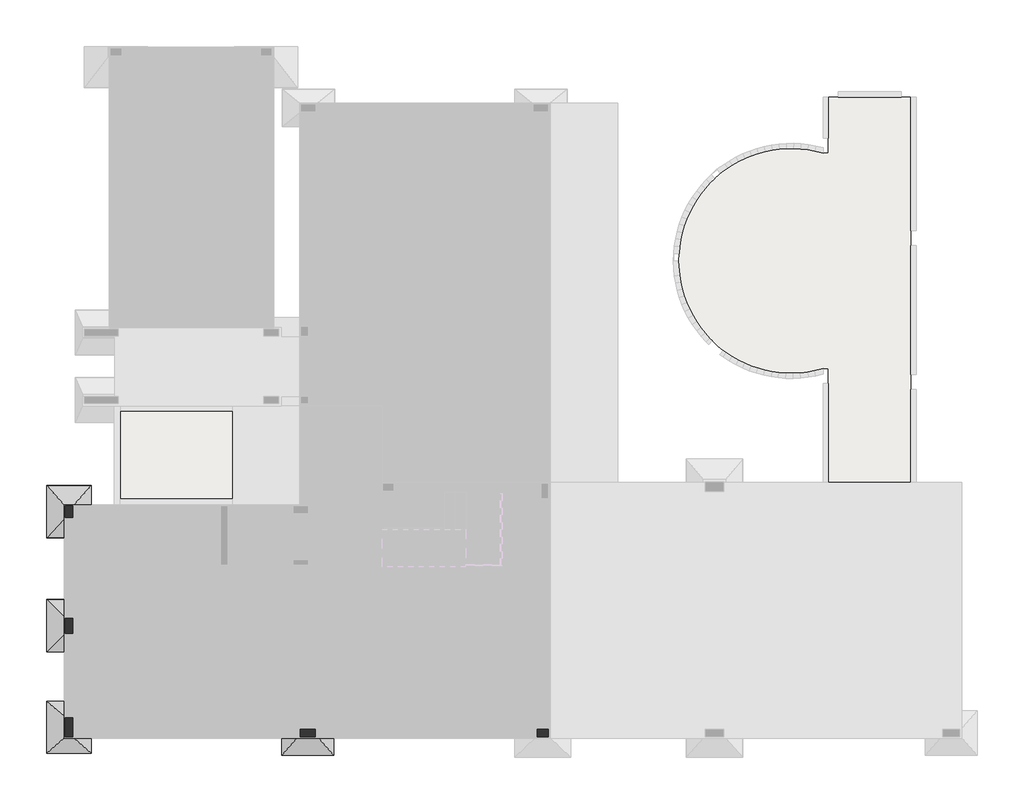
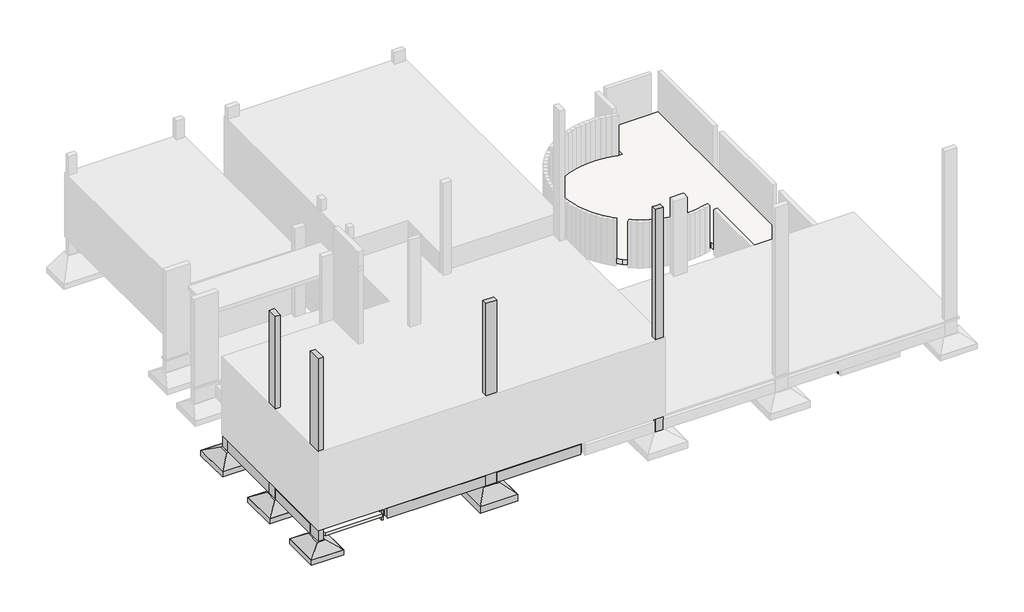
# One storey, part 1 of 4: 11 beams, 5 columns, 4 fasteners, 3 slabs.
# Revit data of these elements (continued)
# Project information
#   Design Option = "Main Model"
#   Project Status = "Status do projeto"
#   Project Address = "RUA SÉRGIO DIAS, LOTE 30, QUADRA G, MONTE MINEIRO/MG"
#   Project Name = "RESIDÊNCIA - ROBERTA VENDRAMINI"
#   Project Number = "034/2017"
#   Zona = "ZER - 01"
#   CA Mín = "0.2"
#   CA Básico = "1"
#   CA Máx = "2"
#   TO Máx = "50"
#   Gabarito Máx = "10"
#   TP Mín = "15"
#   Área Total do Terreno = "620.00 m²"
#   Multifamiliar - Vagas Veículos/Pavto = "0"
#   Multifamiliar - Vagas Bicicletas/Pavto = "0"
#   Multifamiliar - % Vagas PNMR = "0"
#   Multifamiliar - % Vagas Motos = "0"
#   Outros - Área p/ 1 Veículo = "0.00 m²"
#   Outros - Área p/ 1 Bicicleta = "0.00 m²"
#   Outros - Área p/ 1 Utilitário = "0.00 m²"
#   Outros - % Vagas PNMR = "0"
#   Outros - % Vagas Motos = "0"
# Type "TQS - Viga retangular : 14.0 x 40.0"
#   Length [instance default] = 1.524 m
#   b = 0.14 m
#   h = 0.40 m
#   Structural Material [instance default] = none
#   Assembly Code = ""
# Type "TQS - Viga retangular : 19.0 x 40.0"
#   Length [instance default] = 1.524 m
#   b = 0.19 m
#   h = 0.40 m
#   Structural Material [instance default] = none
#   Assembly Code = ""
# Type "TQS - Viga retangular : 19.0 x 55.0"
#   Length [instance default] = 1.524 m
#   b = 0.19 m
#   h = 0.55 m
#   Structural Material [instance default] = none
#   Assembly Code = ""
# Type "TQS - Pilar retangular : 19.0 x 30.0"
#   b = 0.19 m
#   h = 0.30 m
#   Structural Material [instance default] = Concrete - Cast-in-Place Concrete
# Type "TQS - Pilar retangular : 19.0 x 40.0"
#   b = 0.19 m
#   h = 0.40 m
#   Structural Material [instance default] = Concrete - Cast-in-Place Concrete
# Type "TQS - Pilar retangular : 19.0 x 50.0"
#   b = 0.19 m
#   h = 0.50 m
#   Structural Material [instance default] = Concrete - Cast-in-Place Concrete
# Type "TQS - Sapata : S15"
#   TY = 0.40 m
#   TX = 0.29 m
#   HS = 0.50 m
#   H0 = 0.20 m
#   EXCYABS = 0.70 m
#   EXCY = 0.00 m
#   EXCXABS = 0.60 m
#   EXCX = 0.00 m
#   DIMY = 1.40 m
#   DIMX = 1.20 m
#   Material estrutural = Concreto - Concreto concretado no local
#   Width = 0
#   Length = 0
# Type "TQS - Sapata : S19"
#   TY = 0.50 m
#   TX = 0.29 m
#   HS = 0.50 m
#   H0 = 0.20 m
#   EXCYABS = 0.70 m
#   EXCY = 0.00 m
#   EXCXABS = 0.60 m
#   EXCX = 0.00 m
#   DIMY = 1.40 m
#   DIMX = 1.20 m
#   Material estrutural = Concreto - Concreto concretado no local
#   Width = 0
#   Length = 0
# Type "TQS - Sapata : S20"
#   TY = 0.60 m
#   TX = 0.29 m
#   HS = 0.50 m
#   H0 = 0.20 m
#   EXCYABS = 0.70 m
#   EXCY = 0.00 m
#   EXCXABS = 0.60 m
#   EXCX = 0.00 m
#   DIMY = 1.40 m
#   DIMX = 1.20 m
#   Material estrutural = Concreto - Concreto concretado no local
#   Width = 0
#   Length = 0
# Type "TQS - Sapata : S21"
#   TY = 0.60 m
#   TX = 0.29 m
#   HS = 0.60 m
#   H0 = 0.25 m
#   EXCYABS = 0.70 m
#   EXCY = 0.00 m
#   EXCXABS = 0.60 m
#   EXCX = 0.00 m
#   DIMY = 1.40 m
#   DIMX = 1.20 m
#   Material estrutural = Concreto - Concreto concretado no local
#   Width = 0
#   Length = 0
# Type "TQS h=12"
#   Function = 0
#   Layers, outside or top first: 0.12 m ".MATERIAL GENÉRICO LAJE E PISO" (function 1)
# Type "TQS h=20"
#   Function = 0
#   Layers, outside or top first: 0.20 m ".MATERIAL GENÉRICO LAJE E PISO" (function 1)
# Element 1 (IfcBeam, "TQS - Viga retangular : 14.0 x 40.0")
#   Uso = "ESTRUTURA"
#   Titulo = "V22"
#   Chave = "-203"
#   Tipo Elemento = "Viga"
#   SHA1 = "0EE0F179185C4FE731D9B7F49CC743500D79D063"
#   Revisão = ""
#   Tipo de carga = ""
#   Divisor de flexao = ""
#   Secao = ""
#   Configuracao = ""
#   Angulo (graus) = ""
#   Detalhamento = ""
#   Casos de vento manual = ""
#   Tipo = ""
#   Alcas = ""
#   Furos = ""
#   Pino = ""
#   Distribuicao = ""
#   Solidarizado = ""
#   Solidarizar na montagem = ""
#   Unir com o próximo = ""
#   Grupo pre moldado = ""
#   Verificado = ""
#   Concreto C = ""
#   Taxa de armadura (kgf/m³) = 0
#   Carga (tf/m²) = 0
#   Carga (tf/m) = 0
#   Carga (tf) = 0
#   Altura = 0.40 m
#   Rebaixo = 0.07 m
#   Largura = 0.14 m
#   Distancia a face = 0.00 m
#   Distancia ao eixo = 0.00 m
#   Altura gerber esquerda = 0.00 m
#   Largura gerber esquerda = 0.00 m
#   Altura gerber direita = 0.00 m
#   Largura gerber direita = 0.00 m
#   Resultado de Ensaios fck (MPa) = 0
#   Unique TQS ID = -203
#   Principal = yes
#   Structural Material = none
#   Phase Created = CC_AP/ESTR
# Element 2 (IfcBeam, "TQS - Viga retangular : 14.0 x 40.0")
#   Uso = "ESTRUTURA"
#   Titulo = "V9"
#   Chave = "-204"
#   Tipo Elemento = "Viga"
#   SHA1 = "AA57A5F4D00ABE88C47FF187D940E0A6D8A99B36"
#   Revisão = ""
#   Tipo de carga = ""
#   Divisor de flexao = ""
#   Secao = ""
#   Configuracao = ""
#   Angulo (graus) = ""
#   Detalhamento = ""
#   Casos de vento manual = ""
#   Tipo = ""
#   Alcas = ""
#   Furos = ""
#   Pino = ""
#   Distribuicao = ""
#   Solidarizado = ""
#   Solidarizar na montagem = ""
#   Unir com o próximo = ""
#   Grupo pre moldado = ""
#   Verificado = ""
#   Concreto C = ""
#   Taxa de armadura (kgf/m³) = 0
#   Carga (tf/m²) = 0
#   Carga (tf/m) = 0
#   Carga (tf) = 0
#   Altura = 0.40 m
#   Rebaixo = 0.07 m
#   Largura = 0.14 m
#   Distancia a face = 0.00 m
#   Distancia ao eixo = 0.00 m
#   Altura gerber esquerda = 0.00 m
#   Largura gerber esquerda = 0.00 m
#   Altura gerber direita = 0.00 m
#   Largura gerber direita = 0.00 m
#   Resultado de Ensaios fck (MPa) = 0
#   Unique TQS ID = -204
#   Principal = yes
#   Structural Material = none
#   Phase Created = CC_AP/ESTR
# Element 3 (IfcBeam, "TQS - Viga retangular : 14.0 x 40.0")
#   Uso = "ESTRUTURA"
#   Titulo = "V9"
#   Chave = "-205"
#   Tipo Elemento = "Viga"
#   SHA1 = "E87C8EEF9F202EE39708C04CA286767B11167BA7"
#   Revisão = ""
#   Tipo de carga = ""
#   Divisor de flexao = ""
#   Secao = ""
#   Configuracao = ""
#   Angulo (graus) = ""
#   Detalhamento = ""
#   Casos de vento manual = ""
#   Tipo = ""
#   Alcas = ""
#   Furos = ""
#   Pino = ""
#   Distribuicao = ""
#   Solidarizado = ""
#   Solidarizar na montagem = ""
#   Unir com o próximo = ""
#   Grupo pre moldado = ""
#   Verificado = ""
#   Concreto C = ""
#   Taxa de armadura (kgf/m³) = 0
#   Carga (tf/m²) = 0
#   Carga (tf/m) = 0
#   Carga (tf) = 0
#   Altura = 0.40 m
#   Rebaixo = 0.07 m
#   Largura = 0.14 m
#   Distancia a face = 0.00 m
#   Distancia ao eixo = 0.00 m
#   Altura gerber esquerda = 0.00 m
#   Largura gerber esquerda = 0.00 m
#   Altura gerber direita = 0.00 m
#   Largura gerber direita = 0.00 m
#   Resultado de Ensaios fck (MPa) = 0
#   Unique TQS ID = -205
#   Principal = yes
#   Structural Material = none
#   Phase Created = CC_AP/ESTR
# Element 4 (IfcBeam, "TQS - Viga retangular : 14.0 x 40.0")
#   Uso = "ESTRUTURA"
#   Titulo = "V18"
#   Chave = "-208"
#   Tipo Elemento = "Viga"
#   SHA1 = "7D362067162B3A08BECFB8E1D38DC108435A0D97"
#   Revisão = ""
#   Tipo de carga = ""
#   Divisor de flexao = ""
#   Secao = ""
#   Configuracao = ""
#   Angulo (graus) = ""
#   Detalhamento = ""
#   Casos de vento manual = ""
#   Tipo = ""
#   Alcas = ""
#   Furos = ""
#   Pino = ""
#   Distribuicao = ""
#   Solidarizado = ""
#   Solidarizar na montagem = ""
#   Unir com o próximo = ""
#   Grupo pre moldado = ""
#   Verificado = ""
#   Concreto C = ""
#   Taxa de armadura (kgf/m³) = 0
#   Carga (tf/m²) = 0
#   Carga (tf/m) = 0
#   Carga (tf) = 0
#   Altura = 0.40 m
#   Rebaixo = 0.07 m
#   Largura = 0.14 m
#   Distancia a face = 0.00 m
#   Distancia ao eixo = 0.00 m
#   Altura gerber esquerda = 0.00 m
#   Largura gerber esquerda = 0.00 m
#   Altura gerber direita = 0.00 m
#   Largura gerber direita = 0.00 m
#   Resultado de Ensaios fck (MPa) = 0
#   Unique TQS ID = -208
#   Principal = yes
#   Structural Material = none
#   Phase Created = CC_AP/ESTR
# Element 5 (IfcBeam, "TQS - Viga retangular : 14.0 x 40.0")
#   Uso = "ESTRUTURA"
#   Titulo = "V11"
#   Chave = "-212"
#   Tipo Elemento = "Viga"
#   SHA1 = "085A6152135AC5E0DDDC9306F8DBF004F37A3D7F"
#   Revisão = ""
#   Tipo de carga = ""
#   Divisor de flexao = ""
#   Secao = ""
#   Configuracao = ""
#   Angulo (graus) = ""
#   Detalhamento = ""
#   Casos de vento manual = ""
#   Tipo = ""
#   Alcas = ""
#   Furos = ""
#   Pino = ""
#   Distribuicao = ""
#   Solidarizado = ""
#   Solidarizar na montagem = ""
#   Unir com o próximo = ""
#   Grupo pre moldado = ""
#   Verificado = ""
#   Concreto C = ""
#   Taxa de armadura (kgf/m³) = 0
#   Carga (tf/m²) = 0
#   Carga (tf/m) = 0
#   Carga (tf) = 0
#   Altura = 0.40 m
#   Rebaixo = 0.07 m
#   Largura = 0.14 m
#   Distancia a face = 0.00 m
#   Distancia ao eixo = 0.00 m
#   Altura gerber esquerda = 0.00 m
#   Largura gerber esquerda = 0.00 m
#   Altura gerber direita = 0.00 m
#   Largura gerber direita = 0.00 m
#   Resultado de Ensaios fck (MPa) = 0
#   Unique TQS ID = -212
#   Principal = yes
#   Structural Material = none
#   Phase Created = CC_AP/ESTR
# Element 6 (IfcBeam, "TQS - Viga retangular : 14.0 x 40.0")
#   Uso = "ESTRUTURA"
#   Titulo = "V25"
#   Chave = "-214"
#   Tipo Elemento = "Viga"
#   SHA1 = "AA587B3825EEEC75667AA8C6AA5AB994AEC66271"
#   Revisão = ""
#   Tipo de carga = ""
#   Divisor de flexao = ""
#   Secao = ""
#   Configuracao = ""
#   Angulo (graus) = ""
#   Detalhamento = ""
#   Casos de vento manual = ""
#   Tipo = ""
#   Alcas = ""
#   Furos = ""
#   Pino = ""
#   Distribuicao = ""
#   Solidarizado = ""
#   Solidarizar na montagem = ""
#   Unir com o próximo = ""
#   Grupo pre moldado = ""
#   Verificado = ""
#   Concreto C = ""
#   Taxa de armadura (kgf/m³) = 0
#   Carga (tf/m²) = 0
#   Carga (tf/m) = 0
#   Carga (tf) = 0
#   Altura = 0.40 m
#   Rebaixo = 0.16 m
#   Largura = 0.14 m
#   Distancia a face = 0.00 m
#   Distancia ao eixo = 0.00 m
#   Altura gerber esquerda = 0.00 m
#   Largura gerber esquerda = 0.00 m
#   Altura gerber direita = 0.00 m
#   Largura gerber direita = 0.00 m
#   Resultado de Ensaios fck (MPa) = 0
#   Unique TQS ID = -214
#   Principal = yes
#   Structural Material = none
#   Phase Created = CC_AP/ESTR
# Element 7 (IfcBeam, "TQS - Viga retangular : 14.0 x 40.0")
#   Uso = "ESTRUTURA"
#   Titulo = "V12"
#   Chave = "-453"
#   Tipo Elemento = "Viga"
#   SHA1 = "D9CD6F477F2EF098F4AC3262D940A040C72B7E2B"
#   Revisão = ""
#   Tipo de carga = ""
#   Divisor de flexao = ""
#   Secao = ""
#   Configuracao = ""
#   Angulo (graus) = ""
#   Detalhamento = ""
#   Casos de vento manual = ""
#   Tipo = ""
#   Alcas = ""
#   Furos = ""
#   Pino = ""
#   Distribuicao = ""
#   Solidarizado = ""
#   Solidarizar na montagem = ""
#   Unir com o próximo = ""
#   Grupo pre moldado = ""
#   Verificado = ""
#   Concreto C = ""
#   Taxa de armadura (kgf/m³) = 0
#   Carga (tf/m²) = 0
#   Carga (tf/m) = 0
#   Carga (tf) = 0
#   Altura = 0.40 m
#   Rebaixo = 0.16 m
#   Largura = 0.14 m
#   Distancia a face = 0.00 m
#   Distancia ao eixo = 0.00 m
#   Altura gerber esquerda = 0.00 m
#   Largura gerber esquerda = 0.00 m
#   Altura gerber direita = 0.00 m
#   Largura gerber direita = 0.00 m
#   Resultado de Ensaios fck (MPa) = 0
#   Unique TQS ID = -453
#   Principal = yes
#   Structural Material = none
#   Phase Created = CC_AP/ESTR
# Element 8 (IfcBeam, "TQS - Viga retangular : 14.0 x 40.0")
#   Uso = "ESTRUTURA"
#   Titulo = "V13"
#   Chave = "-681"
#   Tipo Elemento = "Viga"
#   SHA1 = "E52B93A2F47D403CA690CD63769ABDF0E8B6050A"
#   Revisão = ""
#   Tipo de carga = ""
#   Divisor de flexao = ""
#   Secao = ""
#   Configuracao = ""
#   Angulo (graus) = ""
#   Detalhamento = ""
#   Casos de vento manual = ""
#   Tipo = ""
#   Alcas = ""
#   Furos = ""
#   Pino = ""
#   Distribuicao = ""
#   Solidarizado = ""
#   Solidarizar na montagem = ""
#   Unir com o próximo = ""
#   Grupo pre moldado = ""
#   Verificado = ""
#   Concreto C = ""
#   Taxa de armadura (kgf/m³) = 0
#   Carga (tf/m²) = 0
#   Carga (tf/m) = 0
#   Carga (tf) = 0
#   Altura = 0.40 m
#   Rebaixo = 0.07 m
#   Largura = 0.14 m
#   Distancia a face = 0.00 m
#   Distancia ao eixo = 0.00 m
#   Altura gerber esquerda = 0.00 m
#   Largura gerber esquerda = 0.00 m
#   Altura gerber direita = 0.00 m
#   Largura gerber direita = 0.00 m
#   Resultado de Ensaios fck (MPa) = 0
#   Unique TQS ID = -681
#   Principal = yes
#   Structural Material = none
#   Phase Created = CC_AP/ESTR
# Element 9 (IfcBeam, "TQS - Viga retangular : 19.0 x 40.0")
#   Uso = "ESTRUTURA"
#   Titulo = "V16"
#   Chave = "-181"
#   Tipo Elemento = "Viga"
#   SHA1 = "AC6EE286E954C664F8248081444A5D98129228D8"
#   Revisão = ""
#   Tipo de carga = ""
#   Divisor de flexao = ""
#   Secao = ""
#   Configuracao = ""
#   Angulo (graus) = ""
#   Detalhamento = ""
#   Casos de vento manual = ""
#   Tipo = ""
#   Alcas = ""
#   Furos = ""
#   Pino = ""
#   Distribuicao = ""
#   Solidarizado = ""
#   Solidarizar na montagem = ""
#   Unir com o próximo = ""
#   Grupo pre moldado = ""
#   Verificado = ""
#   Concreto C = ""
#   Taxa de armadura (kgf/m³) = 0
#   Carga (tf/m²) = 0
#   Carga (tf/m) = 0
#   Carga (tf) = 0
#   Altura = 0.40 m
#   Rebaixo = 0.07 m
#   Largura = 0.19 m
#   Distancia a face = 0.00 m
#   Distancia ao eixo = 0.00 m
#   Altura gerber esquerda = 0.00 m
#   Largura gerber esquerda = 0.00 m
#   Altura gerber direita = 0.00 m
#   Largura gerber direita = 0.00 m
#   Resultado de Ensaios fck (MPa) = 0
#   Unique TQS ID = -181
#   Principal = yes
#   Structural Material = none
#   Phase Created = CC_AP/ESTR
# Element 10 (IfcBeam, "TQS - Viga retangular : 19.0 x 40.0")
#   Uso = "ESTRUTURA"
#   Titulo = "V14"
#   Chave = "-188"
#   Tipo Elemento = "Viga"
#   SHA1 = "7A53358B50FB0481EBEA1D15A12D2A0FCC9FC715"
#   Revisão = ""
#   Tipo de carga = ""
#   Divisor de flexao = ""
#   Secao = ""
#   Configuracao = ""
#   Angulo (graus) = ""
#   Detalhamento = ""
#   Casos de vento manual = ""
#   Tipo = ""
#   Alcas = ""
#   Furos = ""
#   Pino = ""
#   Distribuicao = ""
#   Solidarizado = ""
#   Solidarizar na montagem = ""
#   Unir com o próximo = ""
#   Grupo pre moldado = ""
#   Verificado = ""
#   Concreto C = ""
#   Taxa de armadura (kgf/m³) = 0
#   Carga (tf/m²) = 0
#   Carga (tf/m) = 0
#   Carga (tf) = 0
#   Altura = 0.40 m
#   Rebaixo = 0.07 m
#   Largura = 0.19 m
#   Distancia a face = 0.00 m
#   Distancia ao eixo = 0.00 m
#   Altura gerber esquerda = 0.00 m
#   Largura gerber esquerda = 0.00 m
#   Altura gerber direita = 0.00 m
#   Largura gerber direita = 0.00 m
#   Resultado de Ensaios fck (MPa) = 0
#   Unique TQS ID = -188
#   Principal = yes
#   Structural Material = none
#   Phase Created = CC_AP/ESTR
# Element 11 (IfcBeam, "TQS - Viga retangular : 19.0 x 55.0")
#   Uso = "ESTRUTURA"
#   Titulo = "V7"
#   Chave = "-184"
#   Tipo Elemento = "Viga"
#   SHA1 = "E9EC7280BBA3FFEC13DD100B26C6CC66CFF47B76"
#   Revisão = ""
#   Tipo de carga = ""
#   Divisor de flexao = ""
#   Secao = ""
#   Configuracao = ""
#   Angulo (graus) = ""
#   Detalhamento = ""
#   Casos de vento manual = ""
#   Tipo = ""
#   Alcas = ""
#   Furos = ""
#   Pino = ""
#   Distribuicao = ""
#   Solidarizado = ""
#   Solidarizar na montagem = ""
#   Unir com o próximo = ""
#   Grupo pre moldado = ""
#   Verificado = ""
#   Concreto C = ""
#   Taxa de armadura (kgf/m³) = 0
#   Carga (tf/m²) = 0
#   Carga (tf/m) = 0
#   Carga (tf) = 0
#   Altura = 0.55 m
#   Rebaixo = 0.07 m
#   Largura = 0.19 m
#   Distancia a face = 0.00 m
#   Distancia ao eixo = 0.00 m
#   Altura gerber esquerda = 0.00 m
#   Largura gerber esquerda = 0.00 m
#   Altura gerber direita = 0.00 m
#   Largura gerber direita = 0.00 m
#   Resultado de Ensaios fck (MPa) = 0
#   Unique TQS ID = -184
#   Principal = yes
#   Structural Material = none
#   Phase Created = CC_AP/ESTR
# Element 12 (IfcColumn, "TQS - Pilar retangular : 19.0 x 30.0")
#   Uso = "ESTRUTURA"
#   Titulo = "P22"
#   Chave = "P22//0"
#   Tipo Elemento = "Pilar"
#   SHA1 = "74B32C051183367140A14ED156F148A997E93745"
#   Revisão = ""
#   Tipo de carga = ""
#   Divisor de flexao = ""
#   Secao = "R 19/30 90°"
#   Configuracao = ""
#   Angulo (graus) = ""
#   Detalhamento = ""
#   Casos de vento manual = ""
#   Tipo = ""
#   Alcas = ""
#   Furos = ""
#   Pino = ""
#   Distribuicao = ""
#   Solidarizado = ""
#   Solidarizar na montagem = ""
#   Unir com o próximo = ""
#   Grupo pre moldado = ""
#   Verificado = ""
#   Concreto C = ""
#   Taxa de armadura (kgf/m³) = 0
#   Carga (tf/m²) = 0
#   Carga (tf/m) = 0
#   Carga (tf) = 0
#   Altura = 8.25 m
#   Rebaixo = 0.00 m
#   Altura da fundacao = 0.00 m
#   Largura = 0.00 m
#   Distancia a face = 0.00 m
#   Distancia ao eixo = 0.00 m
#   Resultado de Ensaios fck (MPa) = 0
#   Unique TQS ID = -52
#   Principal = yes
#   Nasce = yes
#   Morre = yes
#   Cabeca de Pilar = no
#   Structural Material = Concrete - Cast-in-Place Concrete
#   Phase Created = CC_AP/ESTR
#   Materials on its faces: "Concrete - Cast-in-Place Concrete"
# Element 13 (IfcColumn, "TQS - Pilar retangular : 19.0 x 30.0")
#   Uso = "ESTRUTURA"
#   Titulo = "P15"
#   Chave = "P15//0"
#   Tipo Elemento = "Pilar"
#   SHA1 = "E1EF40F284DB4178944633D19F269044313D4902"
#   Revisão = ""
#   Tipo de carga = ""
#   Divisor de flexao = ""
#   Secao = "R 19/30"
#   Configuracao = ""
#   Angulo (graus) = ""
#   Detalhamento = ""
#   Casos de vento manual = ""
#   Tipo = ""
#   Alcas = ""
#   Furos = ""
#   Pino = ""
#   Distribuicao = ""
#   Solidarizado = ""
#   Solidarizar na montagem = ""
#   Unir com o próximo = ""
#   Grupo pre moldado = ""
#   Verificado = ""
#   Concreto C = ""
#   Taxa de armadura (kgf/m³) = 0
#   Carga (tf/m²) = 0
#   Carga (tf/m) = 0
#   Carga (tf) = 0
#   Altura = 3.10 m
#   Rebaixo = 0.00 m
#   Altura da fundacao = 0.00 m
#   Largura = 0.00 m
#   Distancia a face = 0.00 m
#   Distancia ao eixo = 0.00 m
#   Resultado de Ensaios fck (MPa) = 0
#   Unique TQS ID = -165
#   Principal = yes
#   Nasce = yes
#   Morre = yes
#   Cabeca de Pilar = no
#   Structural Material = Concrete - Cast-in-Place Concrete
#   Phase Created = CC_AP/ESTR
#   Materials on its faces: "Concrete - Cast-in-Place Concrete"
# Element 14 (IfcColumn, "TQS - Pilar retangular : 19.0 x 40.0")
#   Uso = "ESTRUTURA"
#   Titulo = "P19"
#   Chave = "P19//0"
#   Tipo Elemento = "Pilar"
#   SHA1 = "093B358AFDBAA251B04AA547A5D91A122216BA95"
#   Revisão = ""
#   Tipo de carga = ""
#   Divisor de flexao = ""
#   Secao = "R 19/40"
#   Configuracao = ""
#   Angulo (graus) = ""
#   Detalhamento = ""
#   Casos de vento manual = ""
#   Tipo = ""
#   Alcas = ""
#   Furos = ""
#   Pino = ""
#   Distribuicao = ""
#   Solidarizado = ""
#   Solidarizar na montagem = ""
#   Unir com o próximo = ""
#   Grupo pre moldado = ""
#   Verificado = ""
#   Concreto C = ""
#   Taxa de armadura (kgf/m³) = 0
#   Carga (tf/m²) = 0
#   Carga (tf/m) = 0
#   Carga (tf) = 0
#   Altura = 6.15 m
#   Rebaixo = 0.00 m
#   Altura da fundacao = 0.00 m
#   Largura = 0.00 m
#   Distancia a face = 0.00 m
#   Distancia ao eixo = 0.00 m
#   Resultado de Ensaios fck (MPa) = 0
#   Unique TQS ID = -55
#   Principal = yes
#   Nasce = yes
#   Morre = yes
#   Cabeca de Pilar = no
#   Structural Material = Concrete - Cast-in-Place Concrete
#   Phase Created = CC_AP/ESTR
#   Materials on its faces: "Concrete - Cast-in-Place Concrete"
# Element 15 (IfcColumn, "TQS - Pilar retangular : 19.0 x 40.0")
#   Uso = "ESTRUTURA"
#   Titulo = "P21"
#   Chave = "P21//0"
#   Tipo Elemento = "Pilar"
#   SHA1 = "7EA026137CEA6DD5128C297612ADEF5773B66F62"
#   Revisão = ""
#   Tipo de carga = ""
#   Divisor de flexao = ""
#   Secao = "R 19/40 270°"
#   Configuracao = ""
#   Angulo (graus) = ""
#   Detalhamento = ""
#   Casos de vento manual = ""
#   Tipo = ""
#   Alcas = ""
#   Furos = ""
#   Pino = ""
#   Distribuicao = ""
#   Solidarizado = ""
#   Solidarizar na montagem = ""
#   Unir com o próximo = ""
#   Grupo pre moldado = ""
#   Verificado = ""
#   Concreto C = ""
#   Taxa de armadura (kgf/m³) = 0
#   Carga (tf/m²) = 0
#   Carga (tf/m) = 0
#   Carga (tf) = 0
#   Altura = 6.15 m
#   Rebaixo = 0.00 m
#   Altura da fundacao = 0.00 m
#   Largura = 0.00 m
#   Distancia a face = 0.00 m
#   Distancia ao eixo = 0.00 m
#   Resultado de Ensaios fck (MPa) = 0
#   Unique TQS ID = -166
#   Principal = yes
#   Nasce = yes
#   Morre = yes
#   Cabeca de Pilar = no
#   Structural Material = Concrete - Cast-in-Place Concrete
#   Phase Created = CC_AP/ESTR
#   Materials on its faces: "Concrete - Cast-in-Place Concrete"
# Element 16 (IfcColumn, "TQS - Pilar retangular : 19.0 x 50.0")
#   Uso = "ESTRUTURA"
#   Titulo = "P20"
#   Chave = "P20//0"
#   Tipo Elemento = "Pilar"
#   SHA1 = "CBA1581784D1834A270D99BD43DC7DB390139A31"
#   Revisão = ""
#   Tipo de carga = ""
#   Divisor de flexao = ""
#   Secao = "R 19/50"
#   Configuracao = ""
#   Angulo (graus) = ""
#   Detalhamento = ""
#   Casos de vento manual = ""
#   Tipo = ""
#   Alcas = ""
#   Furos = ""
#   Pino = ""
#   Distribuicao = ""
#   Solidarizado = ""
#   Solidarizar na montagem = ""
#   Unir com o próximo = ""
#   Grupo pre moldado = ""
#   Verificado = ""
#   Concreto C = ""
#   Taxa de armadura (kgf/m³) = 0
#   Carga (tf/m²) = 0
#   Carga (tf/m) = 0
#   Carga (tf) = 0
#   Altura = 6.15 m
#   Rebaixo = 0.00 m
#   Altura da fundacao = 0.00 m
#   Largura = 0.00 m
#   Distancia a face = 0.00 m
#   Distancia ao eixo = 0.00 m
#   Resultado de Ensaios fck (MPa) = 0
#   Unique TQS ID = -54
#   Principal = yes
#   Nasce = yes
#   Morre = yes
#   Cabeca de Pilar = no
#   Structural Material = Concrete - Cast-in-Place Concrete
#   Phase Created = CC_AP/ESTR
#   Materials on its faces: "Concrete - Cast-in-Place Concrete"
# Element 17 (IfcFastener, "TQS - Sapata : S15")
#   Uso = "ESTRUTURA"
#   Titulo = "S15"
#   Chave = "-1472"
#   Tipo Elemento = "Fundação"
#   SHA1 = "D4CAB0671F7DE7F29C2B2445B1EEE28D1894D6FF"
#   Revisão = ""
#   Tipo de carga = ""
#   Divisor de flexao = ""
#   Secao = ""
#   Configuracao = ""
#   Angulo (graus) = ""
#   Detalhamento = ""
#   Casos de vento manual = ""
#   Tipo = "Sapata"
#   Dimensoes = "120.0,140.0"
#   Estacas = ""
#   Calice = ""
#   Rugosidade = ""
#   Alcas = ""
#   Furos = ""
#   Pino = ""
#   Distribuicao = ""
#   Solidarizado = ""
#   Solidarizar na montagem = ""
#   Unir com o próximo = ""
#   Grupo pre moldado = ""
#   Verificado = ""
#   Concreto C = ""
#   Taxa de armadura (kgf/m³) = 0
#   Carga (tf/m²) = 0
#   Carga (tf/m) = 0
#   Carga (tf) = 0
#   Altura = 0.00 m
#   Rebaixo = 0.00 m
#   Pilar ficticio = 0.00 m
#   Topo = 0.03 m
#   Altura total = 0.50 m
#   Rodape = 0.00 m
#   Diametro = 0.00 m
#   Altura dentro do bloco = 0.00 m
#   Entre eixos = 0.00 m
#   Paredes = 0.00 m
#   Caimento = 0.00 m
#   Largura = 0.00 m
#   Distancia a face = 0.00 m
#   Distancia ao eixo = 0.00 m
#   Resultado de Ensaios fck (MPa) = 0
#   Unique TQS ID = -1472
#   Principal = yes
#   Phase Created = CC_AP/ESTR
#   Materials on its faces: "Concreto - Concreto concretado no local"
# Element 18 (IfcFastener, "TQS - Sapata : S19")
#   Uso = "ESTRUTURA"
#   Titulo = "S19"
#   Chave = "-1464"
#   Tipo Elemento = "Fundação"
#   SHA1 = "696692FDA33825790091079D26A0FC1744923CA0"
#   Revisão = ""
#   Tipo de carga = ""
#   Divisor de flexao = ""
#   Secao = ""
#   Configuracao = ""
#   Angulo (graus) = ""
#   Detalhamento = ""
#   Casos de vento manual = ""
#   Tipo = "Sapata"
#   Dimensoes = "120.0,140.0"
#   Estacas = ""
#   Calice = ""
#   Rugosidade = ""
#   Alcas = ""
#   Furos = ""
#   Pino = ""
#   Distribuicao = ""
#   Solidarizado = ""
#   Solidarizar na montagem = ""
#   Unir com o próximo = ""
#   Grupo pre moldado = ""
#   Verificado = ""
#   Concreto C = ""
#   Taxa de armadura (kgf/m³) = 0
#   Carga (tf/m²) = 0
#   Carga (tf/m) = 0
#   Carga (tf) = 0
#   Altura = 0.00 m
#   Rebaixo = 0.00 m
#   Pilar ficticio = 0.00 m
#   Topo = 0.03 m
#   Altura total = 0.50 m
#   Rodape = 0.00 m
#   Diametro = 0.00 m
#   Altura dentro do bloco = 0.00 m
#   Entre eixos = 0.00 m
#   Paredes = 0.00 m
#   Caimento = 0.00 m
#   Largura = 0.00 m
#   Distancia a face = 0.00 m
#   Distancia ao eixo = 0.00 m
#   Resultado de Ensaios fck (MPa) = 0
#   Unique TQS ID = -1464
#   Principal = yes
#   Phase Created = CC_AP/ESTR
#   Materials on its faces: "Concreto - Concreto concretado no local"
# Element 19 (IfcFastener, "TQS - Sapata : S20")
#   Uso = "ESTRUTURA"
#   Titulo = "S20"
#   Chave = "-1462"
#   Tipo Elemento = "Fundação"
#   SHA1 = "E8A55F044D5D0FEDAF3A2E52ADD3CCB0BA977F38"
#   Revisão = ""
#   Tipo de carga = ""
#   Divisor de flexao = ""
#   Secao = ""
#   Configuracao = ""
#   Angulo (graus) = ""
#   Detalhamento = ""
#   Casos de vento manual = ""
#   Tipo = "Sapata"
#   Dimensoes = "120.0,140.0"
#   Estacas = ""
#   Calice = ""
#   Rugosidade = ""
#   Alcas = ""
#   Furos = ""
#   Pino = ""
#   Distribuicao = ""
#   Solidarizado = ""
#   Solidarizar na montagem = ""
#   Unir com o próximo = ""
#   Grupo pre moldado = ""
#   Verificado = ""
#   Concreto C = ""
#   Taxa de armadura (kgf/m³) = 0
#   Carga (tf/m²) = 0
#   Carga (tf/m) = 0
#   Carga (tf) = 0
#   Altura = 0.00 m
#   Rebaixo = 0.00 m
#   Pilar ficticio = 0.00 m
#   Topo = 0.03 m
#   Altura total = 0.50 m
#   Rodape = 0.00 m
#   Diametro = 0.00 m
#   Altura dentro do bloco = 0.00 m
#   Entre eixos = 0.00 m
#   Paredes = 0.00 m
#   Caimento = 0.00 m
#   Largura = 0.00 m
#   Distancia a face = 0.00 m
#   Distancia ao eixo = 0.00 m
#   Resultado de Ensaios fck (MPa) = 0
#   Unique TQS ID = -1462
#   Principal = yes
#   Phase Created = CC_AP/ESTR
#   Materials on its faces: "Concreto - Concreto concretado no local"
# Element 20 (IfcFastener, "TQS - Sapata : S21")
#   Uso = "ESTRUTURA"
#   Titulo = "S21"
#   Chave = "-1463"
#   Tipo Elemento = "Fundação"
#   SHA1 = "0C6532C4A6A661814370FBEABFA2346616E70F6C"
#   Revisão = ""
#   Tipo de carga = ""
#   Divisor de flexao = ""
#   Secao = ""
#   Configuracao = ""
#   Angulo (graus) = ""
#   Detalhamento = ""
#   Casos de vento manual = ""
#   Tipo = "Sapata"
#   Dimensoes = "120.0,140.0"
#   Estacas = ""
#   Calice = ""
#   Rugosidade = ""
#   Alcas = ""
#   Furos = ""
#   Pino = ""
#   Distribuicao = ""
#   Solidarizado = ""
#   Solidarizar na montagem = ""
#   Unir com o próximo = ""
#   Grupo pre moldado = ""
#   Verificado = ""
#   Concreto C = ""
#   Taxa de armadura (kgf/m³) = 0
#   Carga (tf/m²) = 0
#   Carga (tf/m) = 0
#   Carga (tf) = 0
#   Altura = 0.00 m
#   Rebaixo = 0.00 m
#   Pilar ficticio = 0.00 m
#   Topo = 0.03 m
#   Altura total = 0.60 m
#   Rodape = 0.00 m
#   Diametro = 0.00 m
#   Altura dentro do bloco = 0.00 m
#   Entre eixos = 0.00 m
#   Paredes = 0.00 m
#   Caimento = 0.00 m
#   Largura = 0.00 m
#   Distancia a face = 0.00 m
#   Distancia ao eixo = 0.00 m
#   Resultado de Ensaios fck (MPa) = 0
#   Unique TQS ID = -1463
#   Principal = yes
#   Phase Created = CC_AP/ESTR
#   Materials on its faces: "Concreto - Concreto concretado no local"
# Element 21 (IfcSlab, "TQS h=12")
#   Uso = "ESTRUTURA"
#   Titulo = "L2"
#   Chave = "-541"
#   Tipo Elemento = "Laje"
#   SHA1 = "9D88A251886EA259D37D7D6526C24190D18449DE"
#   Revisão = ""
#   Tipo de carga = ""
#   Divisor de flexao = ""
#   Fabricante = ""
#   Enchimento = ""
#   Mini painel = ""
#   Blocos por nervura = ""
#   Secao = ""
#   Configuracao = ""
#   Angulo (graus) = "0"
#   Detalhamento = ""
#   Casos de vento manual = ""
#   Tipo = "Maciça"
#   Alcas = ""
#   Furos = ""
#   Pino = ""
#   Distribuicao = ""
#   Solidarizado = ""
#   Solidarizar na montagem = ""
#   Unir com o próximo = ""
#   Grupo pre moldado = ""
#   Verificado = ""
#   Concreto C = ""
#   Height Offset From Level = -0.50 m
#   Taxa de armadura (kgf/m³) = 0
#   Carga (tf/m²) = 0
#   Carga (tf/m) = 0
#   Carga (tf) = 0
#   Altura = 0.12 m
#   Capa = 0.00 m
#   Capa inferior = 0.00 m
#   Altura da nervura = 0.00 m
#   Enchimento (tf/m³) = 0
#   Largura inferior X = 0.00 m
#   Distancia inferior X = 0.00 m
#   Largura inferior Y = 0.00 m
#   Distancia inferior Y = 0.00 m
#   Largura vigota = 0.00 m
#   Altura vigota = 0.00 m
#   Largura perfil = 0.00 m
#   Largura aba = 0.00 m
#   Altura perfil = 0.00 m
#   Nervura secundaria = 0.00 m
#   Desconto nervura secundaria = 0.00 m
#   Rebaixo = -0.50 m
#   Largura = 0.00 m
#   Distancia a face = 0.00 m
#   Distancia ao eixo = 0.00 m
#   Resultado de Ensaios fck (MPa) = 0
#   built-in parameter 1001954 = 1
#   Unique TQS ID = -541
#   Principal = yes
#   Phase Created = CC_AP/ESTR
#   Materials on its faces: ".MATERIAL GENÉRICO LAJE E PISO"
# Element 22 (IfcSlab, "TQS h=12")
#   Uso = "ESTRUTURA"
#   Titulo = "L8"
#   Chave = "-680"
#   Tipo Elemento = "Laje"
#   SHA1 = "9859310AA961365E5B9659041FB058FECACF80B9"
#   Revisão = ""
#   Tipo de carga = ""
#   Divisor de flexao = ""
#   Fabricante = ""
#   Enchimento = ""
#   Mini painel = ""
#   Blocos por nervura = ""
#   Secao = ""
#   Configuracao = ""
#   Angulo (graus) = "0"
#   Detalhamento = ""
#   Casos de vento manual = ""
#   Tipo = "Maciça"
#   Alcas = ""
#   Furos = ""
#   Pino = ""
#   Distribuicao = ""
#   Solidarizado = ""
#   Solidarizar na montagem = ""
#   Unir com o próximo = ""
#   Grupo pre moldado = ""
#   Verificado = ""
#   Concreto C = ""
#   Height Offset From Level = -0.18 m
#   Taxa de armadura (kgf/m³) = 0
#   Carga (tf/m²) = 0
#   Carga (tf/m) = 0
#   Carga (tf) = 0
#   Altura = 0.12 m
#   Capa = 0.00 m
#   Capa inferior = 0.00 m
#   Altura da nervura = 0.00 m
#   Enchimento (tf/m³) = 0
#   Largura inferior X = 0.00 m
#   Distancia inferior X = 0.00 m
#   Largura inferior Y = 0.00 m
#   Distancia inferior Y = 0.00 m
#   Largura vigota = 0.00 m
#   Altura vigota = 0.00 m
#   Largura perfil = 0.00 m
#   Largura aba = 0.00 m
#   Altura perfil = 0.00 m
#   Nervura secundaria = 0.00 m
#   Desconto nervura secundaria = 0.00 m
#   Rebaixo = -0.18 m
#   Largura = 0.00 m
#   Distancia a face = 0.00 m
#   Distancia ao eixo = 0.00 m
#   Resultado de Ensaios fck (MPa) = 0
#   built-in parameter 1001954 = 1
#   Unique TQS ID = -680
#   Principal = yes
#   Phase Created = CC_AP/ESTR
#   Materials on its faces: ".MATERIAL GENÉRICO LAJE E PISO"
# Element 23 (IfcSlab, "TQS h=20")
#   Uso = "ESTRUTURA"
#   Titulo = "L4"
#   Chave = "-843"
#   Tipo Elemento = "Laje"
#   SHA1 = "FB4864774B549ABE2AC3E52C0811E4BD1C9F7941"
#   Revisão = ""
#   Tipo de carga = ""
#   Divisor de flexao = ""
#   Fabricante = ""
#   Enchimento = ""
#   Mini painel = ""
#   Blocos por nervura = ""
#   Secao = ""
#   Configuracao = ""
#   Angulo (graus) = "0"
#   Detalhamento = ""
#   Casos de vento manual = ""
#   Tipo = "Maciça"
#   Alcas = ""
#   Furos = ""
#   Pino = ""
#   Distribuicao = ""
#   Solidarizado = ""
#   Solidarizar na montagem = ""
#   Unir com o próximo = ""
#   Grupo pre moldado = ""
#   Verificado = ""
#   Concreto C = ""
#   Height Offset From Level = -1.75 m
#   Taxa de armadura (kgf/m³) = 0
#   Carga (tf/m²) = 0
#   Carga (tf/m) = 0
#   Carga (tf) = 0
#   Altura = 0.20 m
#   Capa = 0.00 m
#   Capa inferior = 0.00 m
#   Altura da nervura = 0.00 m
#   Enchimento (tf/m³) = 0
#   Largura inferior X = 0.00 m
#   Distancia inferior X = 0.00 m
#   Largura inferior Y = 0.00 m
#   Distancia inferior Y = 0.00 m
#   Largura vigota = 0.00 m
#   Altura vigota = 0.00 m
#   Largura perfil = 0.00 m
#   Largura aba = 0.00 m
#   Altura perfil = 0.00 m
#   Nervura secundaria = 0.00 m
#   Desconto nervura secundaria = 0.00 m
#   Rebaixo = -1.75 m
#   Largura = 0.00 m
#   Distancia a face = 0.00 m
#   Distancia ao eixo = 0.00 m
#   Resultado de Ensaios fck (MPa) = 0
#   built-in parameter 1001954 = 1
#   Unique TQS ID = -843
#   Principal = yes
#   Phase Created = CC_AP/ESTR
#   Materials on its faces: ".MATERIAL GENÉRICO LAJE E PISO"
# Materials
#   "Concrete - Cast-in-Place Concrete": class "Unassigned", colour RGB 192 192 192, transparency 0
#   "Concreto - Concreto concretado no local": class "Concreto", colour RGB 192 192 192, transparency 0
#   ".MATERIAL GENÉRICO LAJE E PISO": class ".CC_PAVIMENTAÇÃO", colour RGB 128 128 128, transparency 0, Description = "Material genérico para representação ND 200.", Cost = 0
